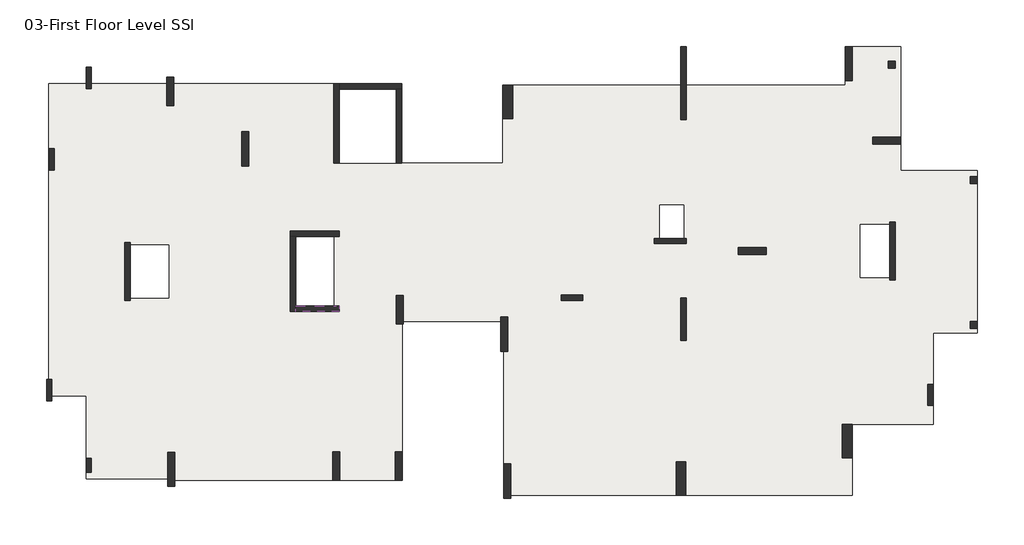
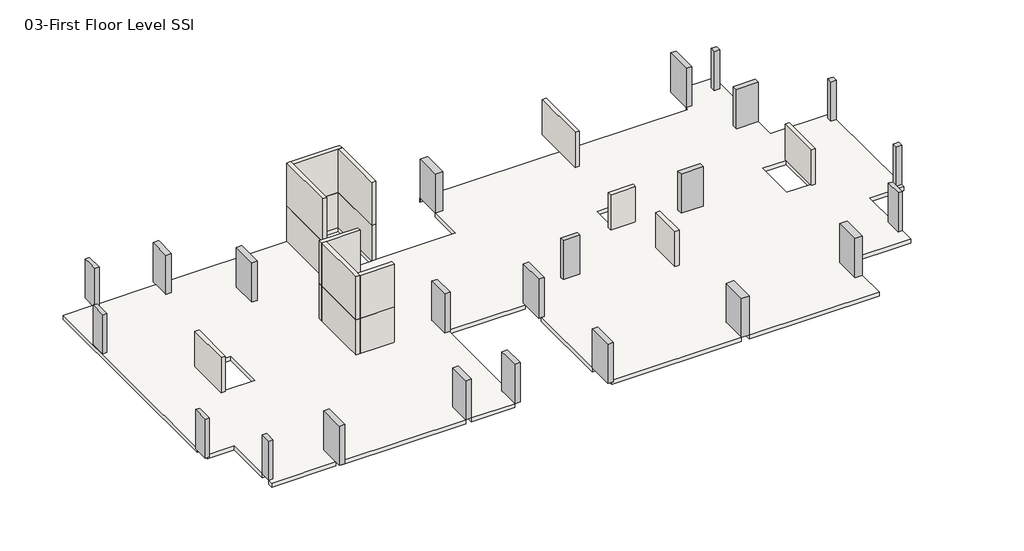
# One storey: 23 columns, 17 walls, 1 slab.
"""IFC4 building model written with IfcOpenShell, lengths in millimetres."""

from ifc_helpers import new_model, si_unit, frame, origin, place, context, project, spatial, polyline, outline, extrude, faceted_brep, element, save

model = new_model("IFC4")

# Units and contexts
model_context = context("Model", 3, world=origin())
ifc_project = project(units=[si_unit("LENGTHUNIT", "METRE", prefix="MILLI")], contexts=[model_context])

# Site, building, storey
site = spatial("IfcSite", under=ifc_project)
building = spatial("IfcBuilding", under=site)
storey = spatial("IfcBuildingStorey", under=building, Name="03-First Floor Level SSl", Elevation=3000.0)

# Columns
placement = place(None, origin())
element("IfcColumn", 1, ObjectType="M_Concrete-Rectangular-Column : C-1 (400 x 400mm)", at=placement, inside=storey, context=model_context, shape_type="Brep", body=[
    faceted_brep([(52549.9999998, 16712.0, 3000.0), (52549.9999998, 16312.0, 3000.0), (52149.9999998, 16312.0, 3000.0), (52149.9999998, 16712.0, 3000.0), (52549.9999998, 16712.0, 6000.0), (52549.9999998, 16312.0, 6000.0), (52549.9999998, 16312.0, 5700.0), (52549.9999998, 16712.0, 5700.0), (52149.9999998, 16312.0, 6000.0), (52149.9999998, 16312.0, 5700.0), (52149.9999998, 16712.0, 6000.0), (52149.9999998, 16712.0, 5700.0)], [[[0, 1, 2, 3]], [[4, 5, 6, 1, 0, 7]], [[5, 8, 9, 2, 1, 6]], [[8, 10, 11, 3, 2, 9]], [[10, 4, 7, 0, 3, 11]], [[4, 10, 8, 5]]]),
])
element("IfcColumn", 2, ObjectType="M_Concrete-Rectangular-Column : C-1 (400 x 400mm)", at=placement, inside=storey, context=model_context, shape_type="Brep", body=[
    faceted_brep([(47898.6337868, 23252.0, 3000.0), (47898.6337868, 22852.0, 3000.0), (47498.6337868, 22852.0, 3000.0), (47498.6337868, 23252.0, 3000.0), (47898.6337868, 23252.0, 6000.0), (47898.6337868, 22852.0, 6000.0), (47898.6337868, 22852.0, 5700.0), (47498.6337868, 22852.0, 6000.0), (47498.6337868, 22852.0, 5700.0), (47498.6337868, 23252.0, 6000.0)], [[[0, 1, 2, 3]], [[4, 5, 6, 1, 0]], [[5, 7, 8, 2, 1, 6]], [[7, 9, 3, 2, 8]], [[9, 4, 0, 3]], [[4, 9, 7, 5]]]),
])
element("IfcColumn", 3, ObjectType="M_Concrete-Rectangular-Column : C-1 (400 x 400mm)", at=placement, inside=storey, context=model_context, shape_type="Brep", body=[
    faceted_brep([(52549.9999998, 8504.0039609, 3000.0), (52549.9999998, 8104.0039609, 3000.0), (52149.9999998, 8104.0039609, 3000.0), (52149.9999998, 8504.0039609, 3000.0), (52549.9999998, 8504.0039609, 6000.0), (52549.9999998, 8104.0039609, 6000.0), (52549.9999998, 8104.0039609, 5700.0), (52549.9999998, 8504.0039609, 5700.0), (52149.9999998, 8104.0039609, 6000.0), (52149.9999998, 8104.0039609, 5700.0), (52149.9999998, 8504.0039609, 6000.0), (52149.9999998, 8504.0039609, 5700.0)], [[[0, 1, 2, 3]], [[4, 5, 6, 1, 0, 7]], [[5, 8, 9, 2, 1, 6]], [[8, 10, 11, 3, 2, 9]], [[10, 4, 7, 0, 3, 11]], [[4, 10, 8, 5]]]),
])
element("IfcColumn", 4, ObjectType="M_Concrete-Rectangular-Column : C-2 (300 x 800mm)", at=placement, inside=storey, context=model_context, shape_type="Brep", body=[
    faceted_brep([(2352.0, 728.0, 3000.0), (2352.0, -72.0, 3000.0), (2052.0, -72.0, 3000.0), (2052.0, 728.0, 3000.0), (2352.0, 728.0, 6000.0), (2352.0, -72.0, 6000.0), (2352.0, -72.0, 5700.0), (2352.0, 728.0, 5700.0), (2052.0, -72.0, 6000.0), (2052.0, -72.0, 5700.0), (2052.0, 728.0, 6000.0), (2052.0, 728.0, 5700.0)], [[[0, 1, 2, 3]], [[4, 5, 6, 1, 0, 7]], [[5, 8, 9, 2, 1, 6]], [[8, 10, 11, 3, 2, 9]], [[10, 4, 7, 0, 3, 11]], [[4, 10, 8, 5]]]),
])
element("IfcColumn", 5, ObjectType="M_Concrete-Rectangular-Column : C-3(300 x 1200mm)", at=placement, inside=storey, context=model_context, shape_type="Brep", body=[
    faceted_brep([(2352.0, 22908.0000656, 3000.0), (2352.0, 21708.0000656, 3000.0), (2052.0, 21708.0000656, 3000.0), (2052.0, 22908.0000656, 3000.0), (2352.0, 22908.0000656, 6000.0), (2352.0, 21708.0000656, 6000.0), (2352.0, 21708.0000656, 5700.0), (2352.0, 22908.0000656, 5700.0), (2052.0, 21708.0000656, 6000.0), (2052.0, 21708.0000656, 5700.0), (2052.0, 22380.0004589, 6000.0), (2052.0, 22908.0000656, 6000.0), (2052.0, 22908.0000656, 5700.0)], [[[0, 1, 2, 3]], [[4, 5, 6, 1, 0, 7]], [[5, 8, 9, 2, 1, 6]], [[8, 10, 11, 12, 3, 2, 9]], [[11, 4, 7, 0, 3, 12]], [[4, 11, 10, 8, 5]]]),
])
element("IfcColumn", 6, ObjectType="M_Concrete-Rectangular-Column : C-3(300 x 1200mm)", at=placement, inside=storey, context=model_context, shape_type="Brep", body=[
    faceted_brep([(257.9999999, 18288.0, 3000.0), (257.9999999, 17088.0, 3000.0), (-42.0000001, 17088.0, 3000.0), (-42.0000001, 18288.0, 3000.0), (257.9999999, 18288.0, 6000.0), (257.9999999, 17088.0, 6000.0), (257.9999999, 17088.0, 5700.0), (257.9999999, 18288.0, 5700.0), (-42.0000001, 17088.0, 6000.0), (-42.0000001, 17088.0, 5700.0), (-42.0000001, 18288.0, 6000.0), (-42.0000001, 18288.0, 5700.0)], [[[0, 1, 2, 3]], [[4, 5, 6, 1, 0, 7]], [[5, 8, 9, 2, 1, 6]], [[8, 10, 11, 3, 2, 9]], [[10, 4, 7, 0, 3, 11]], [[4, 10, 8, 5]]]),
])
element("IfcColumn", 7, ObjectType="M_Concrete-Rectangular-Column : C-3(300 x 1200mm)", at=placement, inside=storey, context=model_context, shape_type="Brep", body=[
    faceted_brep([(108.001803, 5201.9999858, 3000.0), (108.001803, 4001.9999858, 3000.0), (-191.998197, 4001.9999858, 3000.0), (-191.998197, 5201.9999858, 3000.0), (108.001803, 5201.9999858, 6000.0), (108.001803, 4001.9999858, 6000.0), (108.001803, 4001.9999858, 5700.0), (108.001803, 5201.9999858, 5700.0), (-191.998197, 4001.9999858, 6000.0), (-191.998197, 4001.9999858, 5700.0), (-191.998197, 5201.9999858, 6000.0), (-191.998197, 5201.9999858, 5700.0)], [[[0, 1, 2, 3]], [[4, 5, 6, 1, 0, 7]], [[5, 8, 9, 2, 1, 6]], [[8, 10, 11, 3, 2, 9]], [[10, 4, 7, 0, 3, 11]], [[4, 10, 8, 5]]]),
])
element("IfcColumn", 8, ObjectType="M_Concrete-Rectangular-Column : C-3(300 x 1200mm)", at=placement, inside=storey, context=model_context, shape_type="Brep", body=[
    faceted_brep([(50046.0009271, 4931.9999929, 3000.0), (50046.0009271, 3731.9999929, 3000.0), (49746.0009271, 3731.9999929, 3000.0), (49746.0009271, 4931.9999929, 3000.0), (50046.0009271, 4931.9999929, 6000.0), (50046.0009271, 3731.9999929, 6000.0), (50046.0009271, 3731.9999929, 5700.0), (50046.0009271, 4931.9999929, 5700.0), (49746.0009271, 3731.9999929, 6000.0), (49746.0009271, 3731.9999929, 5700.0), (49746.0009271, 4931.9999929, 6000.0), (49746.0009271, 4931.9999929, 5700.0)], [[[0, 1, 2, 3]], [[4, 5, 6, 1, 0, 7]], [[5, 8, 9, 2, 1, 6]], [[8, 10, 11, 3, 2, 9]], [[10, 4, 7, 0, 3, 11]], [[4, 10, 8, 5]]]),
])
element("IfcColumn", 9, ObjectType="M_Concrete-Rectangular-Column : C-3(300 x 1200mm)", at=placement, inside=storey, context=model_context, shape_type="Brep", body=[
    faceted_brep([(28975.9999998, 9996.0000019, 3000.0), (30175.9999998, 9996.0000019, 3000.0), (30175.9999998, 9696.0000019, 3000.0), (28975.9999998, 9696.0000019, 3000.0), (28975.9999998, 9996.0000019, 6000.0), (30175.9999998, 9996.0000019, 6000.0), (30175.9999998, 9996.0000019, 5700.0), (28975.9999998, 9996.0000019, 5700.0), (30175.9999998, 9696.0000019, 6000.0), (30175.9999998, 9696.0000019, 5700.0), (28975.9999998, 9696.0000019, 6000.0), (28975.9999998, 9696.0000019, 5700.0)], [[[0, 1, 2, 3]], [[4, 5, 6, 1, 0, 7]], [[5, 8, 9, 2, 1, 6]], [[8, 10, 11, 3, 2, 9]], [[10, 4, 7, 0, 3, 11]], [[4, 10, 8, 5]]]),
])
element("IfcColumn", 10, ObjectType="M_Concrete-Rectangular-Column : C-4 (400 x 1600mm)", at=placement, inside=storey, context=model_context, shape_type="Brep", body=[
    faceted_brep([(7021.9999999, 22340.0000078, 3000.0), (7021.9999999, 20740.0000078, 3000.0), (6621.9999999, 20740.0000078, 3000.0), (6621.9999999, 22340.0000078, 3000.0), (7021.9999999, 22340.0000078, 6000.0), (7021.9999999, 20740.0000078, 6000.0), (7021.9999999, 20740.0000078, 5700.0), (7021.9999999, 22340.0000078, 5700.0), (6621.9999999, 20740.0000078, 6000.0), (6621.9999999, 20740.0000078, 5700.0), (6621.9999999, 22340.0000078, 6000.0), (6621.9999999, 22340.0000078, 5700.0)], [[[0, 1, 2, 3]], [[4, 5, 6, 1, 0, 7]], [[5, 8, 9, 2, 1, 6]], [[8, 10, 11, 3, 2, 9]], [[10, 4, 7, 0, 3, 11]], [[4, 10, 8, 5]]]),
])
element("IfcColumn", 11, ObjectType="M_Concrete-Rectangular-Column : C-4 (400 x 1600mm)", at=placement, inside=storey, context=model_context, shape_type="Brep", body=[
    faceted_brep([(19969.9997488, 1087.9955348, 3000.0), (19969.9997488, -512.0044652, 3000.0), (19569.9997488, -512.0044652, 3000.0), (19569.9997488, 1087.9955348, 3000.0), (19969.9997488, 1087.9955348, 6000.0), (19969.9997488, -512.0044652, 6000.0), (19969.9997488, -512.0044652, 5700.0), (19969.9997488, 1087.9955348, 5700.0), (19569.9997488, -512.0044652, 6000.0), (19569.9997488, -512.0044652, 5700.0), (19569.9997488, 564.000519, 6000.0), (19569.9997488, 1087.9955348, 6000.0), (19569.9997488, 1087.9955348, 5700.0)], [[[0, 1, 2, 3]], [[4, 5, 6, 1, 0, 7]], [[5, 8, 9, 2, 1, 6]], [[8, 10, 11, 12, 3, 2, 9]], [[11, 4, 7, 0, 3, 12]], [[4, 11, 10, 8, 5]]]),
])
element("IfcColumn", 12, ObjectType="M_Concrete-Rectangular-Column : C-4 (400 x 1600mm)", at=placement, inside=storey, context=model_context, shape_type="Brep", body=[
    faceted_brep([(46605.9993605, 18950.0, 3000.0), (48205.9993605, 18950.0, 3000.0), (48205.9993605, 18550.0, 3000.0), (46605.9993605, 18550.0, 3000.0), (46605.9993605, 18950.0, 6000.0), (48205.9993605, 18950.0, 6000.0), (48205.9993605, 18950.0, 5700.0), (46605.9993605, 18950.0, 5700.0), (48205.9993605, 18550.0, 6000.0), (48205.9993605, 18550.0, 5700.0), (46605.9993605, 18550.0, 6000.0), (46605.9993605, 18550.0, 5700.0)], [[[0, 1, 2, 3]], [[4, 5, 6, 1, 0, 7]], [[5, 8, 9, 2, 1, 6]], [[8, 10, 11, 3, 2, 9]], [[10, 4, 7, 0, 3, 11]], [[4, 10, 8, 5]]]),
])
element("IfcColumn", 13, ObjectType="M_Concrete-Rectangular-Column : C-5 (400 x 1600mm)", at=placement, inside=storey, context=model_context, shape_type="Brep", body=[
    faceted_brep([(20030.000009, 9955.9999979, 3000.0), (20030.000009, 8355.9999979, 3000.0), (19630.000009, 8355.9999979, 3000.0), (19630.000009, 9955.9999979, 3000.0), (20030.000009, 9955.9999979, 6000.0), (20030.000009, 8355.9999979, 6000.0), (20030.000009, 8355.9999979, 5700.0), (20030.000009, 9955.9999979, 5700.0), (19630.000009, 8355.9999979, 6000.0), (19630.000009, 8355.9999979, 5700.0), (19630.000009, 9955.9999979, 6000.0), (19630.000009, 9955.9999979, 5700.0)], [[[0, 1, 2, 3]], [[4, 5, 6, 1, 0, 7]], [[5, 8, 9, 2, 1, 6]], [[8, 10, 11, 3, 2, 9]], [[10, 4, 7, 0, 3, 11]], [[4, 10, 8, 5]]]),
])
element("IfcColumn", 14, ObjectType="M_Concrete-Rectangular-Column : C-5 (400 x 1600mm)", at=placement, inside=storey, context=model_context, shape_type="Brep", body=[
    faceted_brep([(16429.9999981, 1088.0, 3000.0), (16429.9999981, -512.0, 3000.0), (16029.9999981, -512.0, 3000.0), (16029.9999981, 1088.0, 3000.0), (16429.9999981, 1088.0, 6000.0), (16429.9999981, 564.000519, 6000.0), (16429.9999981, -512.0, 6000.0), (16429.9999981, -512.0, 5700.0), (16429.9999981, 1088.0, 5700.0), (16029.9999981, -512.0, 6000.0), (16029.9999981, -512.0, 5700.0), (16029.9999981, 1088.0, 6000.0), (16029.9999981, 1088.0, 5700.0)], [[[0, 1, 2, 3]], [[4, 5, 6, 7, 1, 0, 8]], [[6, 9, 10, 2, 1, 7]], [[9, 11, 12, 3, 2, 10]], [[11, 4, 8, 0, 3, 12]], [[4, 11, 9, 6, 5]]]),
])
element("IfcColumn", 15, ObjectType="M_Concrete-Rectangular-Column : C-5 (400 x 1600mm)", at=placement, inside=storey, context=model_context, shape_type="Brep", body=[
    faceted_brep([(38998.0014887, 12692.0079212, 3000.0), (40598.0014887, 12692.0079212, 3000.0), (40598.0014887, 12292.0079212, 3000.0), (38998.0014887, 12292.0079212, 3000.0), (38998.0014887, 12692.0079212, 6000.0), (40598.0014887, 12692.0079212, 6000.0), (40598.0014887, 12692.0079212, 5700.0), (38998.0014887, 12692.0079212, 5700.0), (40598.0014887, 12292.0079212, 6000.0), (40598.0014887, 12292.0079212, 5700.0), (38998.0014887, 12292.0079212, 6000.0), (38998.0014887, 12292.0079212, 5700.0)], [[[0, 1, 2, 3]], [[4, 5, 6, 1, 0, 7]], [[5, 8, 9, 2, 1, 6]], [[8, 10, 11, 3, 2, 9]], [[10, 4, 7, 0, 3, 11]], [[4, 10, 8, 5]]]),
])
element("IfcColumn", 16, ObjectType="M_Concrete-Rectangular-Column : C-6 (400 x 1950mm)", at=placement, inside=storey, context=model_context, shape_type="Brep", body=[
    faceted_brep([(11270.0000427, 19262.9999996, 3000.0), (11270.0000427, 17312.9999996, 3000.0), (10870.0000427, 17312.9999996, 3000.0), (10870.0000427, 19262.9999996, 3000.0), (11270.0000427, 19262.9999996, 6000.0), (11270.0000427, 17312.9999996, 6000.0), (11270.0000427, 17312.9999996, 5700.0), (11270.0000427, 19262.9999996, 5700.0), (10870.0000427, 17312.9999996, 6000.0), (10870.0000427, 17312.9999996, 5700.0), (10870.0000427, 19262.9999996, 6000.0), (10870.0000427, 19262.9999996, 5700.0)], [[[0, 1, 2, 3]], [[4, 5, 6, 1, 0, 7]], [[5, 8, 9, 2, 1, 6]], [[8, 10, 11, 3, 2, 9]], [[10, 4, 7, 0, 3, 11]], [[4, 10, 8, 5]]]),
])
element("IfcColumn", 17, ObjectType="M_Concrete-Rectangular-Column : C-6 (400 x 1950mm)", at=placement, inside=storey, context=model_context, shape_type="Brep", body=[
    faceted_brep([(7082.0000416, 1083.0000153, 3000.0), (7082.0000416, -866.9999847, 3000.0), (6682.0000416, -866.9999847, 3000.0), (6682.0000416, 1083.0000153, 3000.0), (7082.0000416, 1083.0000153, 6000.0), (7082.0000416, -866.9999847, 6000.0), (7082.0000416, -866.9999847, 5700.0), (7082.0000416, 1083.0000153, 5700.0), (6682.0000416, -866.9999847, 6000.0), (6682.0000416, -866.9999847, 5700.0), (6682.0000416, 1083.0000153, 6000.0), (6682.0000416, 1083.0000153, 5700.0)], [[[0, 1, 2, 3]], [[4, 5, 6, 1, 0, 7]], [[5, 8, 9, 2, 1, 6]], [[8, 10, 11, 3, 2, 9]], [[10, 4, 7, 0, 3, 11]], [[4, 10, 8, 5]]]),
])
element("IfcColumn", 18, ObjectType="M_Concrete-Rectangular-Column : C-6 (400 x 1950mm)", at=placement, inside=storey, context=model_context, shape_type="Brep", body=[
    faceted_brep([(26113.9999998, 422.995535, 3000.0), (26113.9999998, -1527.004465, 3000.0), (25713.9999998, -1527.004465, 3000.0), (25713.9999998, 422.995535, 3000.0), (26113.9999998, 422.995535, 6000.0), (26113.9999998, -1527.004465, 6000.0), (26113.9999998, -1527.004465, 5700.0), (26113.9999998, 422.995535, 5700.0), (25713.9999998, -1527.004465, 6000.0), (25713.9999998, -1527.004465, 5700.0), (25713.9999998, 422.995535, 6000.0), (25713.9999998, 422.995535, 5700.0)], [[[0, 1, 2, 3]], [[4, 5, 6, 1, 0, 7]], [[5, 8, 9, 2, 1, 6]], [[8, 10, 11, 3, 2, 9]], [[10, 4, 7, 0, 3, 11]], [[4, 10, 8, 5]]]),
])
element("IfcColumn", 19, ObjectType="M_Concrete-Rectangular-Column : C-6 (400 x 1950mm)", at=placement, inside=storey, context=model_context, shape_type="Brep", body=[
    faceted_brep([(45446.0007483, 24087.0, 3000.0), (45446.0007483, 22137.0, 3000.0), (45046.0007483, 22137.0, 3000.0), (45046.0007483, 24087.0, 3000.0), (45446.0007483, 24087.0, 6000.0), (45446.0007483, 23252.0000315, 6000.0), (45446.0007483, 22137.0, 6000.0), (45446.0007483, 22137.0, 5700.0), (45446.0007483, 24087.0, 5700.0), (45046.0007483, 22137.0, 6000.0), (45046.0007483, 22137.0, 5700.0), (45046.0007483, 24087.0, 6000.0), (45046.0007483, 24087.0, 5700.0)], [[[0, 1, 2, 3]], [[4, 5, 6, 7, 1, 0, 8]], [[6, 9, 10, 2, 1, 7]], [[9, 11, 12, 3, 2, 10]], [[11, 4, 8, 0, 3, 12]], [[4, 11, 9, 6, 5]]]),
])
element("IfcColumn", 20, ObjectType="M_Concrete-Rectangular-Column : C-6 (400 x 1950mm)", at=placement, inside=storey, context=model_context, shape_type="Brep", body=[
    faceted_brep([(25934.0000455, 8751.0001824, 3000.0), (25934.0000455, 6801.0001824, 3000.0), (25534.0000455, 6801.0001824, 3000.0), (25534.0000455, 8751.0001824, 3000.0), (25934.0000455, 8751.0001824, 6000.0), (25934.0000455, 6801.0001824, 6000.0), (25934.0000455, 6801.0001824, 5700.0), (25934.0000455, 8751.0001824, 5700.0), (25534.0000455, 6801.0001824, 6000.0), (25534.0000455, 6801.0001824, 5700.0), (25534.0000455, 8751.0001824, 6000.0), (25534.0000455, 8751.0001824, 5700.0)], [[[0, 1, 2, 3]], [[4, 5, 6, 1, 0, 7]], [[5, 8, 9, 2, 1, 6]], [[8, 10, 11, 3, 2, 9]], [[10, 4, 7, 0, 3, 11]], [[4, 10, 8, 5]]]),
])
element("IfcColumn", 21, ObjectType="M_Concrete-Rectangular-Column : C-7 (550 x 1900mm)", at=placement, inside=storey, context=model_context, shape_type="Brep", body=[
    faceted_brep([(36035.9999998, 548.0007983, 3000.0), (36035.9999998, -1351.9992017, 3000.0), (35485.9999998, -1351.9992017, 3000.0), (35485.9999998, 548.0007983, 3000.0), (36035.9999998, 548.0007983, 6000.0), (36035.9999998, -1351.9992017, 6000.0), (36035.9999998, -1351.9992017, 5700.0), (36035.9999998, 548.0007983, 5700.0), (35485.9999998, -1351.9992017, 6000.0), (35485.9999998, -1351.9992017, 5700.0), (35485.9999998, 548.0007983, 6000.0), (35485.9999998, 548.0007983, 5700.0)], [[[0, 1, 2, 3]], [[4, 5, 6, 1, 0, 7]], [[5, 8, 9, 2, 1, 6]], [[8, 10, 11, 3, 2, 9]], [[10, 4, 7, 0, 3, 11]], [[4, 10, 8, 5]]]),
])
element("IfcColumn", 22, ObjectType="M_Concrete-Rectangular-Column : C-7 (550 x 1900mm)", at=placement, inside=storey, context=model_context, shape_type="Brep", body=[
    faceted_brep([(45443.9999998, 2648.0, 3000.0), (45443.9999998, 748.0, 3000.0), (44893.9999998, 748.0, 3000.0), (44893.9999998, 2648.0, 3000.0), (45443.9999998, 2648.0, 6000.0), (45443.9999998, 748.0, 6000.0), (45443.9999998, 748.0, 5700.0), (45443.9999998, 2648.0, 5700.0), (44893.9999998, 748.0, 6000.0), (44893.9999998, 748.0, 5700.0), (44893.9999998, 2648.0, 6000.0), (44893.9999998, 2648.0, 5700.0)], [[[0, 1, 2, 3]], [[4, 5, 6, 1, 0, 7]], [[5, 8, 9, 2, 1, 6]], [[8, 10, 11, 3, 2, 9]], [[10, 4, 7, 0, 3, 11]], [[4, 10, 8, 5]]]),
])
element("IfcColumn", 23, ObjectType="M_Concrete-Rectangular-Column : C-7 (550 x 1900mm)", at=placement, inside=storey, context=model_context, shape_type="Brep", body=[
    faceted_brep([(26218.9999998, 21900.0, 3000.0), (26218.9999998, 20000.0, 3000.0), (25668.9999998, 20000.0, 3000.0), (25668.9999998, 21900.0, 3000.0), (26218.9999998, 21900.0, 6000.0), (26218.9999998, 20000.0, 6000.0), (26218.9999998, 20000.0, 5700.0), (26218.9999998, 21900.0, 5700.0), (25668.9999998, 20000.0, 6000.0), (25668.9999998, 20000.0, 5700.0), (25668.9999998, 21900.0, 6000.0), (25668.9999998, 21900.0, 5700.0)], [[[0, 1, 2, 3]], [[4, 5, 6, 1, 0, 7]], [[5, 8, 9, 2, 1, 6]], [[8, 10, 11, 3, 2, 9]], [[10, 4, 7, 0, 3, 11]], [[4, 10, 8, 5]]]),
])

# Slab
element("IfcSlab", 24, ObjectType="Generic 300mm", at=placement, inside=storey, context=model_context, shape_type="Brep", body=[
    faceted_brep([(6682.0000416, -432.0, 2700.0), (2052.0035458, -432.0, 2700.0), (2052.0035458, -72.0, 2700.0), (2352.0, -72.0, 2700.0), (2352.0, 728.0, 2700.0), (2052.0035458, 728.0, 2700.0), (2052.0035458, 4271.9999858, 2700.0), (108.001803, 4271.9999858, 2700.0), (108.001803, 5201.9999858, 2700.0), (-71.9964081, 5201.9999858, 2700.0), (-71.9964081, 21972.0, 2700.0), (2052.0, 21972.0, 2700.0), (2052.0, 21708.0000656, 2700.0), (2352.0, 21708.0000656, 2700.0), (2352.0, 21972.0, 2700.0), (6621.9999999, 21972.0, 2700.0), (6621.9999999, 20740.0000078, 2700.0), (7021.9999999, 20740.0000078, 2700.0), (7021.9999999, 21972.0, 2700.0), (16079.9999997, 21972.0, 2700.0), (16379.9999997, 21972.0, 2700.0), (19919.9999997, 21972.0, 2700.0), (19919.9999997, 21672.0, 2700.0), (19919.9999997, 17468.0, 2700.0), (25668.9999998, 17468.0, 2700.0), (25668.9999998, 20000.0, 2700.0), (26218.9999998, 20000.0, 2700.0), (26218.9999998, 21900.0, 2700.0), (25668.9999998, 21900.0, 2700.0), (25668.9999998, 21902.0, 2700.0), (45046.0007483, 21902.0, 2700.0), (45046.0007483, 22137.0, 2700.0), (45446.0007483, 22137.0, 2700.0), (45446.0007483, 24087.0, 2700.0), (48205.9993605, 24087.0, 2700.0), (48205.9993605, 18950.0, 2700.0), (46605.9993605, 18950.0, 2700.0), (46605.9993605, 18550.0, 2700.0), (48205.9993605, 18550.0, 2700.0), (48205.9993605, 17048.0, 2700.0), (52549.9999998, 17048.0, 2700.0), (52549.9999998, 16712.0, 2700.0), (52149.9999998, 16712.0, 2700.0), (52149.9999998, 16312.0, 2700.0), (52549.9999998, 16312.0, 2700.0), (52549.9999998, 8504.0039609, 2700.0), (52149.9999998, 8504.0039609, 2700.0), (52149.9999998, 8104.0039609, 2700.0), (52549.9999998, 8104.0039609, 2700.0), (52549.9999998, 7848.0, 2700.0), (50046.0009271, 7848.0, 2700.0), (50046.0009271, 4931.9999929, 2700.0), (49746.0009271, 4931.9999929, 2700.0), (49746.0009271, 3731.9999929, 2700.0), (50046.0009271, 3731.9999929, 2700.0), (50046.0009271, 2648.0, 2700.0), (44893.9999998, 2648.0, 2700.0), (44893.9999998, 748.0, 2700.0), (45443.9999998, 748.0, 2700.0), (45443.9999998, -1351.9992017, 2700.0), (36035.9999998, -1351.9992017, 2700.0), (36035.9999998, 548.0007983, 2700.0), (35485.9999998, 548.0007983, 2700.0), (35485.9999998, -1351.9992017, 2700.0), (26113.9999998, -1351.9992017, 2700.0), (26113.9999998, 422.995535, 2700.0), (25713.9999998, 422.995535, 2700.0), (25713.9999998, 6801.0001824, 2700.0), (25934.0000455, 6801.0001824, 2700.0), (25934.0000455, 8751.0001824, 2700.0), (25534.0000455, 8751.0001824, 2700.0), (25534.0000455, 8496.0001824, 2700.0), (20030.000009, 8496.0001824, 2700.0), (20030.000009, 9955.9999979, 2700.0), (19630.000009, 9955.9999979, 2700.0), (19630.000009, 8355.9999979, 2700.0), (19969.9997488, 8355.9999979, 2700.0), (19969.9997488, 1087.9955348, 2700.0), (19569.9997488, 1087.9955348, 2700.0), (19569.9997488, -512.0, 2700.0), (16429.9999981, -512.0, 2700.0), (16429.9999981, 1088.0, 2700.0), (16029.9999981, 1088.0, 2700.0), (16029.9999981, -512.0, 2700.0), (7082.0000416, -512.0, 2700.0), (7082.0000416, 1083.0000153, 2700.0), (6682.0000416, 1083.0000153, 2700.0), (257.9999999, 17088.0, 2700.0), (257.9999999, 18288.0, 2700.0), (-42.0000001, 18288.0, 2700.0), (-42.0000001, 17088.0, 2700.0), (30175.9999998, 9996.0000019, 2700.0), (28975.9999998, 9996.0000019, 2700.0), (28975.9999998, 9696.0000019, 2700.0), (30175.9999998, 9696.0000019, 2700.0), (11270.0000427, 17312.9999996, 2700.0), (11270.0000427, 19262.9999996, 2700.0), (10870.0000427, 19262.9999996, 2700.0), (10870.0000427, 17312.9999996, 2700.0), (40598.0014887, 12692.0079212, 2700.0), (38998.0014887, 12692.0079212, 2700.0), (38998.0014887, 12292.0079212, 2700.0), (40598.0014887, 12292.0079212, 2700.0), (4548.0000034, 12840.0000003, 2700.0), (4548.0000034, 9840.0000003, 2700.0), (6743.9999995, 9840.0000003, 2700.0), (6743.9999995, 12840.0000003, 2700.0), (47580.0014798, 13992.0079177, 2700.0), (45900.001729, 13992.0079177, 2700.0), (45900.001729, 10992.0079181, 2700.0), (47580.0014798, 10992.0079181, 2700.0), (35904.002157, 15108.0000083, 2700.0), (34548.0015145, 15108.0000083, 2700.0), (34548.0015145, 13199.9999992, 2700.0), (35904.002157, 13199.9999992, 2700.0), (19619.9999997, 21672.0, 2700.0), (16379.9999997, 21672.0, 2700.0), (16379.9999997, 17468.0, 2700.0), (19619.9999997, 17468.0, 2700.0), (16079.9999907, 13320.0000002, 2700.0), (13919.9999907, 13320.0000002, 2700.0), (13919.9999907, 9359.999998, 2700.0), (16079.9999907, 9359.999998, 2700.0), (47898.6337868, 22852.0, 2700.0), (47898.6337868, 23252.0, 2700.0), (47498.6337868, 23252.0, 2700.0), (47498.6337868, 22852.0, 2700.0), (2052.0035458, -432.0, 3000.0), (6682.0000416, -432.0, 3000.0), (6682.0000416, 1083.0000153, 3000.0), (7082.0000416, 1083.0000153, 3000.0), (7082.0000416, -512.0, 3000.0), (16029.9999981, -512.0, 3000.0), (16029.9999981, 1088.0, 3000.0), (16429.9999981, 1088.0, 3000.0), (16429.9999981, -512.0, 3000.0), (19569.9997488, -512.0, 3000.0), (19569.9997488, 1087.9955348, 3000.0), (19969.9997488, 1087.9955348, 3000.0), (19969.9997488, 8355.9999979, 3000.0), (19630.000009, 8355.9999979, 3000.0), (19630.000009, 9955.9999979, 3000.0), (20030.000009, 9955.9999979, 3000.0), (20030.000009, 8496.0001824, 3000.0), (25534.0000455, 8496.0001824, 3000.0), (25534.0000455, 8751.0001824, 3000.0), (25934.0000455, 8751.0001824, 3000.0), (25934.0000455, 6801.0001824, 3000.0), (25713.9999998, 6801.0001824, 3000.0), (25713.9999998, 422.995535, 3000.0), (26113.9999998, 422.995535, 3000.0), (26113.9999998, -1351.9992017, 3000.0), (35485.9999998, -1351.9992017, 3000.0), (35485.9999998, 548.0007983, 3000.0), (36035.9999998, 548.0007983, 3000.0), (36035.9999998, -1351.9992017, 3000.0), (45443.9999998, -1351.9992017, 3000.0), (45443.9999998, 748.0, 3000.0), (44893.9999998, 748.0, 3000.0), (44893.9999998, 2648.0, 3000.0), (45443.9999998, 2648.0, 3000.0), (50046.0009271, 2648.0, 3000.0), (50046.0009271, 3731.9999929, 3000.0), (49746.0009271, 3731.9999929, 3000.0), (49746.0009271, 4931.9999929, 3000.0), (50046.0009271, 4931.9999929, 3000.0), (50046.0009271, 7848.0, 3000.0), (52549.9999998, 7848.0, 3000.0), (52549.9999998, 8104.0039609, 3000.0), (52149.9999998, 8104.0039609, 3000.0), (52149.9999998, 8504.0039609, 3000.0), (52549.9999998, 8504.0039609, 3000.0), (52549.9999998, 16312.0, 3000.0), (52149.9999998, 16312.0, 3000.0), (52149.9999998, 16712.0, 3000.0), (52549.9999998, 16712.0, 3000.0), (52549.9999998, 17048.0, 3000.0), (48205.9993605, 17048.0, 3000.0), (48205.9993605, 18550.0, 3000.0), (46605.9993605, 18550.0, 3000.0), (46605.9993605, 18950.0, 3000.0), (48205.9993605, 18950.0, 3000.0), (48205.9993605, 24087.0, 3000.0), (45446.0007483, 24087.0, 3000.0), (45446.0007483, 22137.0, 3000.0), (45046.0007483, 22137.0, 3000.0), (45046.0007483, 21902.0, 3000.0), (25668.9999998, 21902.0, 3000.0), (25668.9999998, 21900.0, 3000.0), (26218.9999998, 21900.0, 3000.0), (26218.9999998, 20000.0, 3000.0), (25668.9999998, 20000.0, 3000.0), (25668.9999998, 17468.0, 3000.0), (19919.9999997, 17468.0, 3000.0), (19919.9999997, 21672.0, 3000.0), (19919.9999997, 21972.0, 3000.0), (19619.9999997, 21972.0, 3000.0), (16379.9999997, 21972.0, 3000.0), (16079.9999997, 21972.0, 3000.0), (7021.9999999, 21972.0, 3000.0), (7021.9999999, 20740.0000078, 3000.0), (6621.9999999, 20740.0000078, 3000.0), (6621.9999999, 21972.0, 3000.0), (2352.0, 21972.0, 3000.0), (2352.0, 21708.0000656, 3000.0), (2052.0, 21708.0000656, 3000.0), (2052.0, 21972.0, 3000.0), (-71.9964081, 21972.0, 3000.0), (-71.9964081, 5201.9999858, 3000.0), (108.001803, 5201.9999858, 3000.0), (108.001803, 4271.9999858, 3000.0), (2052.0035458, 4271.9999858, 3000.0), (2052.0035458, 728.0, 3000.0), (2352.0, 728.0, 3000.0), (2352.0, -72.0, 3000.0), (2052.0035458, -72.0, 3000.0), (257.9999999, 18288.0, 3000.0), (257.9999999, 17088.0, 3000.0), (-42.0000001, 17088.0, 3000.0), (-42.0000001, 18288.0, 3000.0), (28975.9999998, 9996.0000019, 3000.0), (30175.9999998, 9996.0000019, 3000.0), (30175.9999998, 9696.0000019, 3000.0), (28975.9999998, 9696.0000019, 3000.0), (11270.0000427, 19262.9999996, 3000.0), (11270.0000427, 17312.9999996, 3000.0), (10870.0000427, 17312.9999996, 3000.0), (10870.0000427, 19262.9999996, 3000.0), (38998.0014887, 12692.0079212, 3000.0), (40598.0014887, 12692.0079212, 3000.0), (40598.0014887, 12292.0079212, 3000.0), (38998.0014887, 12292.0079212, 3000.0), (4548.0000034, 9840.0000003, 3000.0), (4548.0000034, 12840.0000003, 3000.0), (6743.9999995, 12840.0000003, 3000.0), (6743.9999995, 9840.0000003, 3000.0), (45900.001729, 13992.0079177, 3000.0), (47580.0014798, 13992.0079177, 3000.0), (47580.0014798, 10992.0079181, 3000.0), (45900.001729, 10992.0079181, 3000.0), (34548.0015145, 15108.0000083, 3000.0), (35904.002157, 15108.0000083, 3000.0), (35904.002157, 13199.9999992, 3000.0), (34548.0015145, 13199.9999992, 3000.0), (13919.9999907, 13320.0000002, 3000.0), (16079.9999907, 13320.0000002, 3000.0), (16079.9999907, 9359.999998, 3000.0), (13919.9999907, 9359.999998, 3000.0), (16379.9999997, 21672.0, 3000.0), (19619.9999997, 21672.0, 3000.0), (19619.9999997, 17468.0, 3000.0), (16379.9999997, 17468.0, 3000.0), (47898.6337868, 23252.0, 3000.0), (47898.6337868, 22852.0, 3000.0), (47498.6337868, 22852.0, 3000.0), (47498.6337868, 23252.0, 3000.0)], [[[0, 1, 2, 3, 4, 5, 6, 7, 8, 9, 10, 11, 12, 13, 14, 15, 16, 17, 18, 19, 20, 21, 22, 23, 24, 25, 26, 27, 28, 29, 30, 31, 32, 33, 34, 35, 36, 37, 38, 39, 40, 41, 42, 43, 44, 45, 46, 47, 48, 49, 50, 51, 52, 53, 54, 55, 56, 57, 58, 59, 60, 61, 62, 63, 64, 65, 66, 67, 68, 69, 70, 71, 72, 73, 74, 75, 76, 77, 78, 79, 80, 81, 82, 83, 84, 85, 86], [87, 88, 89, 90], [91, 92, 93, 94], [95, 96, 97, 98], [99, 100, 101, 102], [103, 104, 105, 106], [107, 108, 109, 110], [111, 112, 113, 114], [115, 116, 117, 118], [119, 120, 121, 122], [123, 124, 125, 126]], [[127, 128, 129, 130, 131, 132, 133, 134, 135, 136, 137, 138, 139, 140, 141, 142, 143, 144, 145, 146, 147, 148, 149, 150, 151, 152, 153, 154, 155, 156, 157, 158, 159, 160, 161, 162, 163, 164, 165, 166, 167, 168, 169, 170, 171, 172, 173, 174, 175, 176, 177, 178, 179, 180, 181, 182, 183, 184, 185, 186, 187, 188, 189, 190, 191, 192, 193, 194, 195, 196, 197, 198, 199, 200, 201, 202, 203, 204, 205, 206, 207, 208, 209, 210, 211, 212, 213, 214, 215], [216, 217, 218, 219], [220, 221, 222, 223], [224, 225, 226, 227], [228, 229, 230, 231], [232, 233, 234, 235], [236, 237, 238, 239], [240, 241, 242, 243], [244, 245, 246, 247], [248, 249, 250, 251], [252, 253, 254, 255]], [[1, 0, 128, 127]], [[1, 127, 215, 2]], [[211, 6, 5, 212]], [[7, 6, 211, 210]], [[8, 7, 210, 209]], [[9, 8, 209, 208]], [[10, 9, 208, 207]], [[10, 207, 206, 11]], [[15, 14, 203, 202]], [[19, 18, 199, 198]], [[21, 20, 19, 198, 197, 196, 195]], [[23, 22, 21, 195, 194, 193]], [[24, 23, 193, 192]], [[24, 192, 191, 25]], [[187, 29, 28, 188]], [[30, 29, 187, 186]], [[185, 31, 30, 186]], [[182, 34, 33, 183]], [[34, 182, 181, 35]], [[177, 39, 38, 178]], [[40, 39, 177, 176]], [[40, 176, 175, 41]], [[167, 49, 48, 168]], [[44, 172, 171, 45]], [[50, 49, 167, 166]], [[50, 166, 165, 51]], [[161, 55, 54, 162]], [[55, 161, 160, 159, 56]], [[59, 58, 157, 156]], [[59, 156, 155, 60]], [[64, 63, 152, 151]], [[148, 67, 66, 149]], [[72, 71, 144, 143]], [[77, 76, 139, 138]], [[80, 79, 136, 135]], [[84, 83, 132, 131]], [[13, 204, 203, 14]], [[204, 13, 12, 205]], [[205, 12, 11, 206]], [[87, 217, 216, 88]], [[217, 87, 90, 218]], [[218, 90, 89, 219]], [[219, 89, 88, 216]], [[53, 163, 162, 54]], [[163, 53, 52, 164]], [[164, 52, 51, 165]], [[91, 221, 220, 92]], [[221, 91, 94, 222]], [[222, 94, 93, 223]], [[223, 93, 92, 220]], [[17, 200, 199, 18]], [[200, 17, 16, 201]], [[201, 16, 15, 202]], [[78, 137, 136, 79]], [[137, 78, 77, 138]], [[180, 36, 35, 181]], [[37, 179, 178, 38]], [[179, 37, 36, 180]], [[142, 73, 72, 143]], [[75, 140, 139, 76]], [[140, 75, 74, 141]], [[141, 74, 73, 142]], [[134, 81, 80, 135]], [[82, 133, 132, 83]], [[133, 82, 81, 134]], [[95, 225, 224, 96]], [[225, 95, 98, 226]], [[226, 98, 97, 227]], [[227, 97, 96, 224]], [[130, 85, 84, 131]], [[86, 129, 128, 0]], [[129, 86, 85, 130]], [[150, 65, 64, 151]], [[65, 150, 149, 66]], [[32, 184, 183, 33]], [[184, 32, 31, 185]], [[99, 229, 228, 100]], [[229, 99, 102, 230]], [[230, 102, 101, 231]], [[231, 101, 100, 228]], [[3, 214, 213, 4]], [[214, 3, 2, 215]], [[4, 213, 212, 5]], [[68, 147, 146, 69]], [[147, 68, 67, 148]], [[70, 145, 144, 71]], [[145, 70, 69, 146]], [[154, 61, 60, 155]], [[62, 153, 152, 63]], [[153, 62, 61, 154]], [[57, 158, 157, 58]], [[158, 57, 56, 159]], [[189, 27, 26, 190]], [[190, 26, 25, 191]], [[27, 189, 188, 28]], [[119, 245, 244, 120]], [[120, 244, 247, 121]], [[121, 247, 246, 122]], [[245, 119, 122, 246]], [[115, 249, 248, 116]], [[116, 248, 251, 117]], [[117, 251, 250, 118]], [[249, 115, 118, 250]], [[103, 233, 232, 104]], [[104, 232, 235, 105]], [[105, 235, 234, 106]], [[233, 103, 106, 234]], [[107, 237, 236, 108]], [[108, 236, 239, 109]], [[109, 239, 238, 110]], [[237, 107, 110, 238]], [[111, 241, 240, 112]], [[112, 240, 243, 113]], [[113, 243, 242, 114]], [[241, 111, 114, 242]], [[43, 173, 172, 44]], [[173, 43, 42, 174]], [[174, 42, 41, 175]], [[123, 253, 252, 124]], [[253, 123, 126, 254]], [[254, 126, 125, 255]], [[255, 125, 124, 252]], [[47, 169, 168, 48]], [[169, 47, 46, 170]], [[170, 46, 45, 171]]]),
])

# Walls
element("IfcWall", 25, ObjectType="Shear Walls 300mm", at=placement, inside=storey, context=model_context, shape_type="Brep", body=[
    faceted_brep([(16379.9999997, 17468.0, 3000.0), (16379.9999997, 21672.0, 3000.0), (16379.9999997, 21972.0, 3000.0), (16379.9999997, 21972.0, 5700.0), (16379.9999997, 21822.0, 5700.0), (16379.9999997, 21672.0, 5700.0), (16379.9999997, 17468.0, 5700.0), (16079.9999997, 17468.0, 3000.0), (16079.9999997, 17468.0, 5700.0), (16079.9999997, 21972.0, 5700.0), (16079.9999997, 21972.0, 3000.0)], [[[0, 1, 2, 3, 4, 5, 6]], [[7, 8, 9, 10]], [[2, 1, 0, 7, 10]], [[0, 6, 8, 7]], [[6, 5, 4, 3, 9, 8]], [[3, 2, 10, 9]]]),
])
element("IfcWall", 26, ObjectType="Shear Walls 300mm", at=placement, inside=storey, context=model_context, shape_type="Brep", body=[
    faceted_brep([(19919.9999997, 21972.0, 3000.0), (16379.9999997, 21972.0, 3000.0), (16379.9999997, 21972.0, 5700.0), (19619.9997365, 21972.0, 5700.0), (19919.9999997, 21972.0, 5700.0), (19919.9999997, 21672.0, 3000.0), (19919.9999997, 21672.0, 5700.0), (19619.9999997, 21672.0, 5700.0), (16379.9999997, 21672.0, 5700.0), (16379.9999997, 21672.0, 3000.0), (19619.9999997, 21672.0, 3000.0), (16379.9999997, 21822.0, 5700.0), (19619.9997365, 21822.0, 5700.0), (19919.9999997, 21822.0, 5700.0)], [[[0, 1, 2, 3, 4]], [[5, 6, 7, 8, 9, 10]], [[1, 0, 5, 10, 9]], [[3, 2, 11, 12]], [[11, 8, 7, 6, 13, 4, 3, 12]], [[2, 1, 9, 8, 11]], [[0, 4, 13, 6, 5]]]),
])
element("IfcWall", 27, ObjectType="Shear Walls 300mm", at=placement, inside=storey, context=model_context, shape_type="SweptSolid", body=[
    extrude(outline(polyline([(19919.9999997, 21672.0), (19919.9999997, 17468.0), (19619.9999997, 17468.0), (19619.9999997, 21672.0), (19919.9999997, 21672.0)])), frame((0.0, 0.0, 3000.0), z_axis=(0.0, 0.0, 1.0), x_axis=(1.0, 0.0, 0.0)), (0.0, 0.0, 1.0), 2700.0),
])
element("IfcWall", 28, ObjectType="Shear Walls 300mm", at=placement, inside=storey, context=model_context, shape_type="Brep", body=[
    faceted_brep([(13619.9999907, 13320.0000002, 3000.0), (13919.9999907, 13320.0000002, 3000.0), (16380.0000168, 13320.0000002, 3000.0), (16380.0000168, 13320.0000002, 5700.0), (13919.9999907, 13320.0000002, 5700.0), (13619.9999907, 13320.0000002, 5700.0), (13619.9999907, 13620.0000002, 3000.0), (13619.9999907, 13620.0000002, 5700.0), (16380.0000168, 13620.0000002, 5700.0), (16380.0000168, 13620.0000002, 3000.0)], [[[0, 1, 2, 3, 4, 5]], [[6, 7, 8, 9]], [[2, 1, 0, 6, 9]], [[3, 2, 9, 8]], [[5, 4, 3, 8, 7]], [[0, 5, 7, 6]]]),
])
element("IfcWall", 29, ObjectType="Shear Walls 300mm", at=placement, inside=storey, context=model_context, shape_type="Brep", body=[
    faceted_brep([(13919.9999907, 9059.999998, 3000.0), (13919.9999907, 9359.999998, 3000.0), (13919.9999907, 13320.0000002, 3000.0), (13919.9999907, 13320.0000002, 5700.0), (13919.9999907, 9359.999998, 5700.0), (13919.9999907, 9059.999998, 5700.0), (13619.9999907, 9059.999998, 3000.0), (13619.9999907, 9059.999998, 5700.0), (13619.9999907, 13320.0000002, 5700.0), (13619.9999907, 13320.0000002, 3000.0)], [[[0, 1, 2, 3, 4, 5]], [[6, 7, 8, 9]], [[2, 1, 0, 6, 9]], [[5, 4, 3, 8, 7]], [[3, 2, 9, 8]], [[0, 5, 7, 6]]]),
])
element("IfcWall", 30, ObjectType="Shear Walls 300mm", at=placement, inside=storey, context=model_context, shape_type="Brep", body=[
    faceted_brep([(16380.0000168, 9359.999998, 3000.0), (16079.9999907, 9359.999998, 3000.0), (13919.9999907, 9359.999998, 3000.0), (13919.9999907, 9359.999998, 5700.0), (16380.0000168, 9359.999998, 5700.0), (16380.0000168, 9059.999998, 3000.0), (16380.0000168, 9059.999998, 5700.0), (13919.9999907, 9059.999998, 5700.0), (13919.9999907, 9059.999998, 3000.0)], [[[0, 1, 2, 3, 4]], [[5, 6, 7, 8]], [[2, 1, 0, 5, 8]], [[0, 4, 6, 5]], [[4, 3, 7, 6]], [[3, 2, 8, 7]]]),
])
element("IfcWall", 31, ObjectType="Shear Walls 300mm", at=placement, inside=storey, context=model_context, shape_type="SweptSolid", body=[
    extrude(outline(polyline([(4548.0000025, 12984.0000001), (4548.0000025, 9696.0), (4248.0000025, 9696.0), (4248.0000025, 12984.0000001), (4548.0000025, 12984.0000001)])), frame((0.0, 0.0, 3000.0), z_axis=(0.0, 0.0, 1.0), x_axis=(1.0, 0.0, 0.0)), (0.0, 0.0, 1.0), 2700.0),
])
element("IfcWall", 32, ObjectType="Shear Walls 300mm", at=placement, inside=storey, context=model_context, shape_type="SweptSolid", body=[
    extrude(outline(polyline([(36048.0015201, 12899.9999992), (34248.0015201, 12899.9999992), (34248.0015201, 13199.9999992), (36048.0015201, 13199.9999992), (36048.0015201, 12899.9999992)])), frame((0.0, 0.0, 3000.0), z_axis=(0.0, 0.0, 1.0), x_axis=(1.0, 0.0, 0.0)), (0.0, 0.0, 1.0), 2700.0),
])
element("IfcWall", 33, ObjectType="Shear Walls 300mm", at=placement, inside=storey, context=model_context, shape_type="SweptSolid", body=[
    extrude(outline(polyline([(35748.0054035, 7428.0000762), (35748.0054035, 9840.0000002), (36048.0054035, 9840.0000002), (36048.0054035, 7428.0000762), (35748.0054035, 7428.0000762)])), frame((0.0, 0.0, 3000.0), z_axis=(0.0, 0.0, 1.0), x_axis=(1.0, 0.0, 0.0)), (0.0, 0.0, 1.0), 2700.0),
])
element("IfcWall", 34, ObjectType="Shear Walls 300mm", at=placement, inside=storey, context=model_context, shape_type="SweptSolid", body=[
    extrude(outline(polyline([(47580.0014811, 10848.0079202), (47580.0014811, 14136.0000002), (47880.0014811, 14136.0000002), (47880.0014811, 10848.0079202), (47580.0014811, 10848.0079202)])), frame((0.0, 0.0, 3000.0), z_axis=(0.0, 0.0, 1.0), x_axis=(1.0, 0.0, 0.0)), (0.0, 0.0, 1.0), 2700.0),
])
element("IfcWall", 35, ObjectType="Shear Walls 300mm", at=placement, inside=storey, context=model_context, shape_type="Brep", body=[
    faceted_brep([(36047.9999998, 19932.0, 3000.0), (36047.9999998, 24072.0078999, 3000.0), (36047.9999998, 24072.0078999, 5700.0), (36047.9999998, 19932.0, 5700.0), (35747.9999998, 19932.0, 3000.0), (35747.9999998, 19932.0, 5700.0), (35747.9999998, 24072.000519, 5700.0), (35747.9999998, 24072.0078999, 3000.0)], [[[0, 1, 2, 3]], [[4, 5, 6, 7]], [[1, 0, 4, 7]], [[2, 1, 7, 6]], [[0, 3, 5, 4]], [[3, 2, 6, 5]]]),
])
element("IfcWall", 36, ObjectType="Shear Walls 300mm", at=placement, inside=storey, context=model_context, shape_type="Brep", body=[
    faceted_brep([(16379.9999997, 17468.0, 3000.0), (16379.9999997, 21672.0, 3000.0), (16379.9999997, 21672.0, 5700.0), (16379.9999997, 21972.0, 5700.0), (16379.9999997, 21972.0, 9000.0), (16379.9999997, 21672.0, 9000.0), (16379.9999997, 17468.0, 9000.0), (16079.9999997, 17468.0, 3000.0), (16079.9999997, 17468.0, 5700.0), (16079.9999997, 17468.0, 6000.0), (16079.9999997, 17468.0, 8700.0), (16079.9999997, 17468.0, 9000.0), (16079.9999997, 21972.0, 9000.0), (16079.9999997, 21972.0, 8700.0), (16079.9999997, 21972.0, 6000.0), (16079.9999997, 21972.0, 5700.0), (16079.9999997, 21672.0, 5700.0), (16079.9999997, 21672.0, 3000.0)], [[[0, 1, 2, 3, 4, 5, 6]], [[7, 8, 9, 10, 11, 12, 13, 14, 15, 16, 17]], [[1, 0, 7, 17]], [[6, 5, 4, 12, 11]], [[0, 6, 11, 10, 9, 8, 7]], [[2, 1, 17, 16]], [[3, 15, 14, 13, 12, 4]], [[15, 3, 2, 16]]]),
])
element("IfcWall", 37, ObjectType="Shear Walls 300mm", at=placement, inside=storey, context=model_context, shape_type="Brep", body=[
    faceted_brep([(19619.9999997, 21972.0, 3000.0), (16379.9999997, 21972.0, 3000.0), (16379.9999997, 21972.0, 5700.0), (16379.9999997, 21972.0, 9000.0), (19619.9997365, 21972.0, 9000.0), (19919.9999997, 21972.0, 9000.0), (19919.9999997, 21972.0, 8700.0), (19919.9999997, 21972.0, 6000.0), (19919.9999997, 21972.0, 5700.0), (19619.9999997, 21972.0, 5700.0), (19619.9999997, 21672.0, 3000.0), (19619.9999997, 21672.0, 5700.0), (19919.9999997, 21672.0, 5700.0), (19919.9999997, 21672.0, 9000.0), (19619.9999997, 21672.0, 9000.0), (16379.9999997, 21672.0, 9000.0), (16379.9999997, 21672.0, 3000.0)], [[[0, 1, 2, 3, 4, 5, 6, 7, 8, 9]], [[10, 11, 12, 13, 14, 15, 16]], [[1, 0, 10, 16]], [[5, 4, 3, 15, 14, 13]], [[0, 9, 11, 10]], [[1, 16, 15, 3, 2]], [[5, 13, 12, 8, 7, 6]], [[8, 12, 11, 9]]]),
])
element("IfcWall", 38, ObjectType="Shear Walls 300mm", at=placement, inside=storey, context=model_context, shape_type="Brep", body=[
    faceted_brep([(19919.9999997, 17468.0, 3000.0), (19919.9999997, 21672.0, 3000.0), (19919.9999997, 21672.0, 5700.0), (19919.9999997, 21672.0, 9000.0), (19919.9999997, 17468.0, 9000.0), (19919.9999997, 17468.0, 8700.0), (19919.9999997, 17468.0, 6000.0), (19919.9999997, 17468.0, 5700.0), (19619.9999997, 17468.0, 3000.0), (19619.9999997, 17468.0, 9000.0), (19619.9999997, 21672.0, 9000.0), (19619.9999997, 21672.0, 3000.0)], [[[0, 1, 2, 3, 4, 5, 6, 7]], [[8, 9, 10, 11]], [[1, 0, 8, 11]], [[4, 3, 10, 9]], [[0, 7, 6, 5, 4, 9, 8]], [[1, 11, 10, 3, 2]]]),
])
element("IfcWall", 39, ObjectType="Shear Walls 300mm", at=placement, inside=storey, context=model_context, shape_type="Brep", body=[
    faceted_brep([(13919.9999907, 13320.0000002, 3000.0), (16079.9999907, 13320.0000002, 3000.0), (16380.0000168, 13320.0000002, 3000.0), (16380.0000168, 13320.0000002, 5700.0), (16380.0000168, 13320.0000002, 6000.0), (16380.0000168, 13320.0000002, 8700.0), (16380.0000168, 13320.0000002, 9000.0), (16079.9999907, 13320.0000002, 9000.0), (13919.9999907, 13320.0000002, 9000.0), (13619.9999907, 13320.0000002, 9000.0), (13619.9999907, 13320.0000002, 5700.0), (13919.9999907, 13320.0000002, 5700.0), (13919.9999907, 13620.0000002, 3000.0), (13919.9999907, 13620.0000002, 5700.0), (13619.9999907, 13620.0000002, 5700.0), (13619.9999907, 13620.0000002, 6000.0), (13619.9999907, 13620.0000002, 8700.0), (13619.9999907, 13620.0000002, 9000.0), (16380.0000168, 13620.0000002, 9000.0), (16380.0000168, 13620.0000002, 8700.0), (16380.0000168, 13620.0000002, 6000.0), (16380.0000168, 13620.0000002, 5700.0), (16380.0000168, 13620.0000002, 3000.0)], [[[0, 1, 2, 3, 4, 5, 6, 7, 8, 9, 10, 11]], [[12, 13, 14, 15, 16, 17, 18, 19, 20, 21, 22]], [[2, 1, 0, 12, 22]], [[6, 5, 4, 3, 2, 22, 21, 20, 19, 18]], [[9, 8, 7, 6, 18, 17]], [[0, 11, 13, 12]], [[9, 17, 16, 15, 14, 10]], [[10, 14, 13, 11]]]),
])
element("IfcWall", 40, ObjectType="Shear Walls 300mm", at=placement, inside=storey, context=model_context, shape_type="Brep", body=[
    faceted_brep([(13919.9999907, 9359.999998, 3000.0), (13919.9999907, 13320.0000002, 3000.0), (13919.9999907, 13320.0000002, 9000.0), (13919.9999907, 9359.999998, 9000.0), (13919.9999907, 9059.999998, 9000.0), (13919.9999907, 9059.999998, 5700.0), (13919.9999907, 9359.999998, 5700.0), (13619.9999907, 9359.999998, 3000.0), (13619.9999907, 9359.999998, 5700.0), (13619.9999907, 9059.999998, 5700.0), (13619.9999907, 9059.999998, 6000.0), (13619.9999907, 9059.999998, 8700.0), (13619.9999907, 9059.999998, 9000.0), (13619.9999907, 13320.0000002, 9000.0), (13619.9999907, 13320.0000002, 5700.0), (13619.9999907, 13320.0000002, 3000.0)], [[[0, 1, 2, 3, 4, 5, 6]], [[7, 8, 9, 10, 11, 12, 13, 14, 15]], [[1, 0, 7, 15]], [[4, 3, 2, 13, 12]], [[0, 6, 8, 7]], [[1, 15, 14, 13, 2]], [[4, 12, 11, 10, 9, 5]], [[5, 9, 8, 6]]]),
])
element("IfcWall", 41, ObjectType="Shear Walls 300mm", at=placement, inside=storey, context=model_context, shape_type="Brep", body=[
    faceted_brep([(13919.9999907, 9359.999998, 9000.0), (16079.9999907, 9359.999998, 9000.0), (16380.0000168, 9359.999998, 9000.0), (16380.0000168, 9359.999998, 8700.0), (16380.0000168, 9359.999998, 6000.0), (16380.0000168, 9359.999998, 5700.0), (16079.9999907, 9359.999998, 5700.0), (13919.9999907, 9359.999998, 5700.0), (16380.0000168, 9059.999998, 9000.0), (13919.9999907, 9059.999998, 9000.0), (13919.9999907, 9059.999998, 5700.0), (16380.0000168, 9059.999998, 5700.0), (16380.0000168, 9059.999998, 6000.0), (16380.0000168, 9059.999998, 8700.0)], [[[0, 1, 2, 3, 4, 5, 6, 7]], [[8, 9, 10, 11, 12, 13]], [[2, 1, 0, 9, 8]], [[2, 8, 13, 12, 11, 5, 4, 3]], [[9, 0, 7, 10]], [[7, 6, 5, 11, 10]]]),
])

save(model, "model.ifc")

# Revit data of these elements
# Type "M_Concrete-Rectangular-Column : C-1 (400 x 400mm)"
#   Type Mark = "C01"
#   b = 400 mm
#   h = 400 mm
#   Structural Material [instance default] = Concrete, Cast-in-Place gray
# Type "M_Concrete-Rectangular-Column : C-2 (300 x 800mm)"
#   Type Mark = "C02"
#   b = 300 mm
#   h = 800 mm
#   Structural Material [instance default] = Concrete, Cast-in-Place gray
# Type "M_Concrete-Rectangular-Column : C-3(300 x 1200mm)"
#   Type Mark = "C03"
#   b = 300 mm
#   h = 1200 mm
#   Structural Material [instance default] = Concrete, Cast-in-Place gray
# Type "M_Concrete-Rectangular-Column : C-4 (400 x 1600mm)"
#   Type Mark = "C04"
#   b = 400 mm
#   h = 1600 mm
#   Structural Material [instance default] = Concrete, Cast-in-Place gray
# Type "M_Concrete-Rectangular-Column : C-5 (400 x 1600mm)"
#   Type Mark = "C05"
#   b = 400 mm
#   h = 1600 mm
#   Structural Material [instance default] = Concrete, Cast-in-Place gray
# Type "M_Concrete-Rectangular-Column : C-6 (400 x 1950mm)"
#   Type Mark = "C06"
#   b = 400 mm
#   h = 1950 mm
#   Structural Material [instance default] = Concrete, Cast-in-Place gray
# Type "M_Concrete-Rectangular-Column : C-7 (550 x 1900mm)"
#   Type Mark = "C07"
#   b = 550 mm
#   h = 1900 mm
#   Structural Material [instance default] = Concrete, Cast-in-Place gray
# Type "Generic 300mm"
#   Function = 0
#   Layers, outside or top first: 300 mm "Concrete-RC" (function 1)
# Type "Shear Walls 300mm"
#   Layers, outside or top first: 300 mm "Concrete-RC" (function 1)
# Elements 1, 2, 3 (IfcColumn, "M_Concrete-Rectangular-Column : C-1 (400 x 400mm)")
#   Structural Material = Concrete-RC
#   Phase Created = New Construction
#   Materials on its faces: "Concrete-RC"
# Element 4 (IfcColumn, "M_Concrete-Rectangular-Column : C-2 (300 x 800mm)")
#   Structural Material = Concrete-RC
#   Phase Created = New Construction
#   Materials on its faces: "Concrete-RC"
# Elements 5, 6, 7, 8, 9 (IfcColumn, "M_Concrete-Rectangular-Column : C-3(300 x 1200mm)")
#   Structural Material = Concrete-RC
#   Phase Created = New Construction
#   Materials on its faces: "Concrete-RC"
# Elements 10, 11, 12 (IfcColumn, "M_Concrete-Rectangular-Column : C-4 (400 x 1600mm)")
#   Structural Material = Concrete-RC
#   Phase Created = New Construction
#   Materials on its faces: "Concrete-RC"
# Elements 13, 14, 15 (IfcColumn, "M_Concrete-Rectangular-Column : C-5 (400 x 1600mm)")
#   Structural Material = Concrete-RC
#   Phase Created = New Construction
#   Materials on its faces: "Concrete-RC"
# Elements 16, 17, 18, 19, 20 (IfcColumn, "M_Concrete-Rectangular-Column : C-6 (400 x 1950mm)")
#   Structural Material = Concrete-RC
#   Phase Created = New Construction
#   Materials on its faces: "Concrete-RC"
# Elements 21, 22, 23 (IfcColumn, "M_Concrete-Rectangular-Column : C-7 (550 x 1900mm)")
#   Structural Material = Concrete-RC
#   Phase Created = New Construction
#   Materials on its faces: "Concrete-RC"
# Element 24 (IfcSlab, "Generic 300mm")
#   Height Offset From Level = 0 mm
#   built-in parameter 1001954 = 1
#   Phase Created = New Construction
#   Materials on its faces: "Concrete-RC"
# Elements 25, 26, 27, 28, 29, 30, 31, 32, 33, 34, 35 (IfcWall, "Shear Walls 300mm")
#   Top Offset = 0 mm
#   Base Offset = 0 mm
#   wall height = 2700 mm
#   Phase Created = New Construction
#   Base Constraint = 03-First Floor Level SSl
#   Top Constraint = 04-Typical Floor Level SSL
#   Materials on its faces: "Concrete-RC"
# Elements 36, 37, 38, 39, 40, 41 (IfcWall, "Shear Walls 300mm")
#   Top Offset = 0 mm
#   Base Offset = 0 mm
#   wall height = 6000 mm
#   Phase Created = New Construction
#   Base Constraint = 03-First Floor Level SSl
#   Top Constraint = 05-Typical Floor Level SSL
#   Materials on its faces: "Concrete-RC"
# Materials
#   "Concrete, Cast-in-Place gray": class "Concrete", colour RGB 192 192 192, transparency 0, Description = "Cast-in-place concrete", Cost = 0
#   "Concrete-RC": class "Concrete", colour RGB 128 128 128, transparency 0, Description = "High strength concrete", Cost = 0
